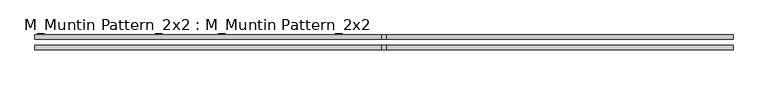
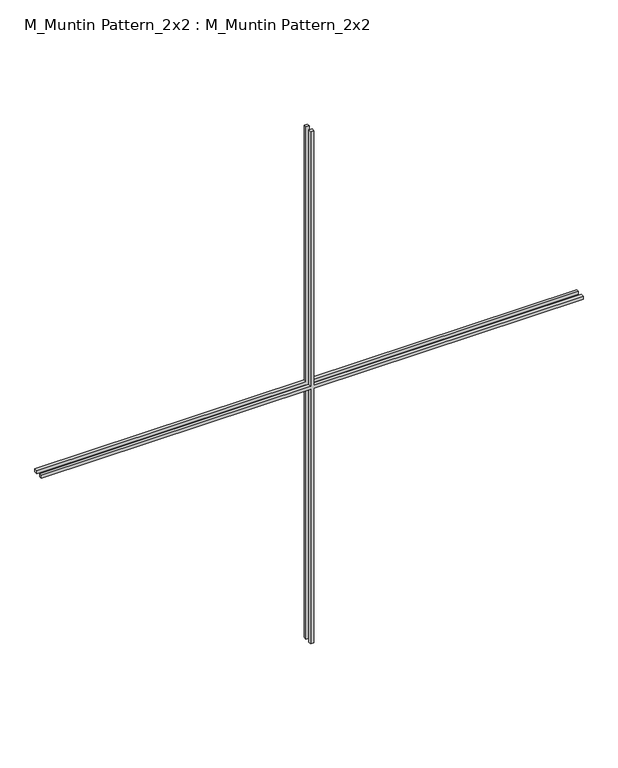
"""IFC4 building model written with IfcOpenShell, lengths in millimetres: proxy geometry, M_Muntin Pattern_2x2 : M_Muntin Pattern_2x2."""

from ifc_helpers import new_model, si_unit, frame, origin, place, context, project, spatial, polyline, outline, extrude, source, transform, mapped, element, save


def m_muntin_pattern_2x2_m_muntin_pattern_2x2_b1a79f21(model_context):
    return source(origin(), model_context, "Body", "SweptSolid", [
        extrude(outline(polyline([(1068.25, -6.35), (1068.25, -1061.9), (1055.55, -1061.9), (1055.55, -6.35), (0.0, -6.35), (0.0, 6.35), (1055.55, 6.35), (1055.55, 1061.9), (1068.25, 1061.9), (1068.25, 6.35), (2123.8, 6.35), (2123.8, -6.35), (1068.25, -6.35)])), frame((0.0, -22.225, 0.0), z_axis=(0.0, 1.0, 0.0), x_axis=(0.0, 0.0, 1.0)), (0.0, 0.0, 1.0), 12.7),
        extrude(outline(polyline([(1068.25, -6.35), (1068.25, -1061.9), (1055.55, -1061.9), (1055.55, -6.35), (0.0, -6.35), (0.0, 6.35), (1055.55, 6.35), (1055.55, 1061.9), (1068.25, 1061.9), (1068.25, 6.35), (2123.8, 6.35), (2123.8, -6.35), (1068.25, -6.35)])), frame((0.0, 9.525, 0.0), z_axis=(0.0, 1.0, 0.0), x_axis=(0.0, 0.0, 1.0)), (0.0, 0.0, 1.0), 12.7),
    ])


if __name__ == "__main__":
    model = new_model("IFC4")
    model_context = context("Model", 3, world=origin())
    ifc_project = project(units=[si_unit("LENGTHUNIT", "METRE", prefix="MILLI")], contexts=[model_context])
    site = spatial("IfcSite", under=ifc_project)
    building = spatial("IfcBuilding", under=site)
    placement = place(None, origin())
    m_muntin_pattern_2x2_m_muntin_pattern_2x2_shape = m_muntin_pattern_2x2_m_muntin_pattern_2x2_b1a79f21(model_context)
    element("IfcBuildingElementProxy", 1, Name="M_Muntin Pattern_2x2 : M_Muntin Pattern_2x2", ObjectType="M_Muntin Pattern_2x2 : M_Muntin Pattern_2x2", at=placement, inside=building, context=model_context, shape_type="MappedRepresentation", body=[
        mapped(m_muntin_pattern_2x2_m_muntin_pattern_2x2_shape, transform((0.0, 0.0, 0.0), x_axis=(1.0, 0.0, 0.0), y_axis=(0.0, 1.0, 0.0), z_axis=(0.0, 0.0, 1.0))),
    ])
    save(model, "model.ifc")

# Revit data of these elements
# Type "M_Muntin Pattern_2x2 : M_Muntin Pattern_2x2"
#   Width [instance default] = 1.20 m
#   Thickness = 0.0127 m
#   Height [instance default] = 1.20 m
#   Distance = 0.01905 m
#   Interior Material [instance default] = none
#   Exterior Material [instance default] = none
#   Default Elevation = 0
# Element 1 (IfcBuildingElementProxy, "M_Muntin Pattern_2x2 : M_Muntin Pattern_2x2")
#   Width = 2.1238 m
#   Height = 2.1238 m
#   Interior Material = Wood - Stained
#   Exterior Material = Clad - White
#   Materials on its faces: "Clad - White", "Wood - Stained"
# Materials
#   "Clad - White": class "Wood", colour RGB 242 242 238, transparency 0, Cost = 0
#   "Wood - Stained": class "Wood", colour RGB 227 170 128, transparency 0, Cost = 0
